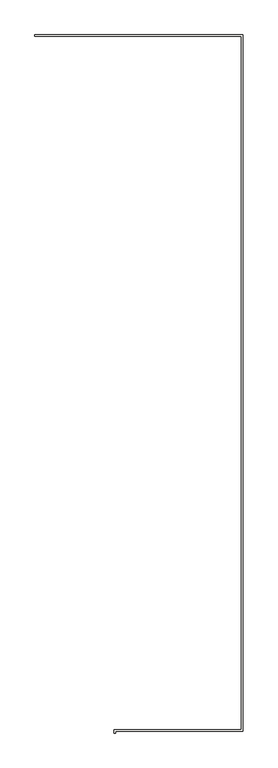
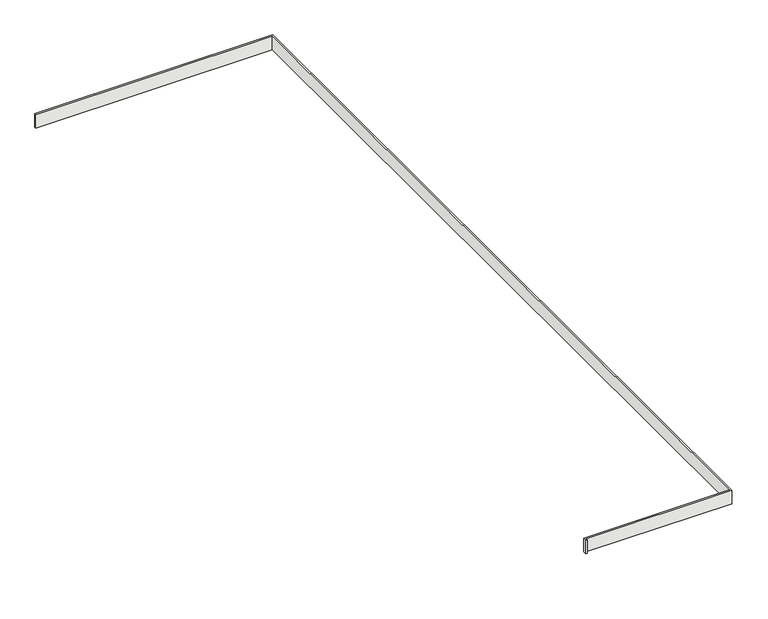
"""IFC4 building model written with IfcOpenShell, lengths in millimetres: slab geometry, FECHAMENTO DECK DE MADEIRA1 : CC_ND 300 FECHAMENTO 2 x 18 cm DECK DE MADEIRA."""

from ifc_helpers import new_model, si_unit, frame, origin, place, context, project, spatial, polyline, outline, extrude, source, transform, mapped, element, save


def slab_ccd32a31(model_context):
    return source(origin(), model_context, "Body", "SweptSolid", [
        extrude(outline(polyline([(11009.718693, -4345.5699847), (10989.718693, -4345.5699847), (10989.718693, -4295.5699847), (12839.718693, -4295.5699847), (12839.718693, 5754.4300153), (9839.718693, 5754.4300153), (9839.718693, 5774.4300153), (12859.718693, 5774.4300153), (12859.718693, -4315.5699847), (11009.718693, -4315.5699847), (11009.718693, -4345.5699847)])), frame((0.0, 0.0, 200.0), z_axis=(0.0, 0.0, 1.0), x_axis=(1.0, 0.0, 0.0)), (0.0, 0.0, 1.0), 180.0),
    ])


if __name__ == "__main__":
    model = new_model("IFC4")
    model_context = context("Model", 3, world=origin())
    ifc_project = project(units=[si_unit("LENGTHUNIT", "METRE", prefix="MILLI")], contexts=[model_context])
    site = spatial("IfcSite", under=ifc_project)
    building = spatial("IfcBuilding", under=site)
    placement = place(None, origin())
    slab_shape = slab_ccd32a31(model_context)
    element("IfcSlab", 1, ObjectType="FECHAMENTO DECK DE MADEIRA1 : CC_ND 300 FECHAMENTO 2 x 18 cm DECK DE MADEIRA", at=placement, inside=building, context=model_context, shape_type="MappedRepresentation", body=[
        mapped(slab_shape, transform((0.0, 0.0, 0.0), x_axis=(1.0, 0.0, 0.0), y_axis=(0.0, 1.0, 0.0), z_axis=(0.0, 0.0, 1.0))),
    ])
    save(model, "model.ifc")

# Revit data of these elements
# Element 1 (IfcSlab, "FECHAMENTO DECK DE MADEIRA1 : CC_ND 300 FECHAMENTO 2 x 18 cm DECK DE MADEIRA")
#   Materials on its faces: ".DECK DE MADEIRA LONGITUDINAL"
# Materials
#   ".DECK DE MADEIRA LONGITUDINAL": class ".CC_MADEIRA REVEST.", colour RGB 169 114 85, transparency 0, Description = "Deck de madeira", Cost = 0
